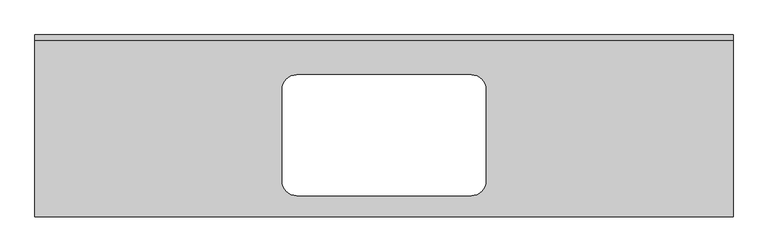
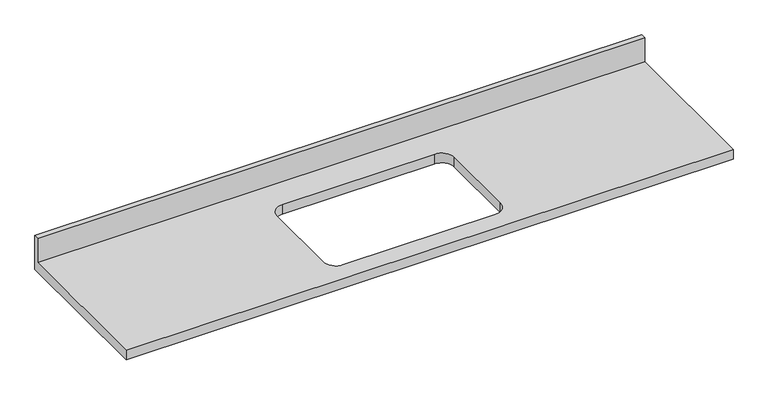
"""IFC4 building model written with IfcOpenShell, lengths in millimetres: furniture geometry, Topo da bancada com pia : Profundidade 600 mm."""

from ifc_helpers import new_model, si_unit, frame, origin, place, context, project, spatial, polyline, circle_curve, source, transform, mapped, element, save
from ifc_brep_helpers import plane_surface, revolved_surface, advanced_brep


def furniture_3e872d23(model_context):
    return source(origin(), model_context, "Body", "AdvancedBrep", [
        advanced_brep(
        [(-1200.4622951, -625.0, 900.0), (1199.5377049, -625.0, 900.0), (1199.5377049, -19.05, 900.0), (-1200.4622951, -19.05, 900.0), (-299.8622951, -137.3, 900.0), (298.9377049, -137.3, 900.0), (349.7377049, -188.1, 900.0), (349.7377049, -501.9, 900.0), (298.9377049, -552.7, 900.0), (-299.8622951, -552.7, 900.0), (-350.6622951, -501.9, 900.0), (-350.6622951, -188.1, 900.0), (1199.5377049, 0.0, 860.0), (1199.5377049, -625.0, 860.0), (-1200.4622951, -625.0, 860.0), (-1200.4622951, 0.0, 860.0), (298.9377049, -137.3, 860.0), (-299.8622951, -137.3, 860.0), (-350.6622951, -188.1, 860.0), (-350.6622951, -501.9, 860.0), (-299.8622951, -552.7, 860.0), (298.9377049, -552.7, 860.0), (349.7377049, -501.9, 860.0), (349.7377049, -188.1, 860.0), (-1200.4622951, 0.0, 1001.6), (1199.5377049, 0.0, 1001.6), (-1200.4622951, -19.05, 1001.6), (1199.5377049, -19.05, 1001.6)],
        [
            (0, 1),
            (1, 2),
            (2, 3),
            (3, 0),
            (4, 5),
            (5, 6, circle_curve(frame((298.9377049, -188.1, 900.0), z_axis=(0.0, 0.0, -1.0), x_axis=(1.0, 0.0, 0.0)), 50.8)),
            (6, 7),
            (7, 8, circle_curve(frame((298.9377049, -501.9, 900.0), z_axis=(0.0, 0.0, -1.0), x_axis=(1.0, 0.0, 0.0)), 50.8)),
            (8, 9),
            (9, 10, circle_curve(frame((-299.8622951, -501.9, 900.0), z_axis=(0.0, 0.0, -1.0), x_axis=(1.0, 0.0, 0.0)), 50.8)),
            (10, 11),
            (11, 4, circle_curve(frame((-299.8622951, -188.1, 900.0), z_axis=(0.0, 0.0, -1.0), x_axis=(1.0, 0.0, 0.0)), 50.8)),
            (12, 13),
            (13, 14),
            (14, 15),
            (15, 12),
            (16, 17),
            (17, 18, circle_curve(frame((-299.8622951, -188.1, 860.0), z_axis=(0.0, 0.0, 1.0), x_axis=(1.0, 0.0, 0.0)), 50.8)),
            (18, 19),
            (19, 20, circle_curve(frame((-299.8622951, -501.9, 860.0), z_axis=(0.0, 0.0, 1.0), x_axis=(1.0, 0.0, 0.0)), 50.8)),
            (20, 21),
            (21, 22, circle_curve(frame((298.9377049, -501.9, 860.0), z_axis=(0.0, 0.0, 1.0), x_axis=(1.0, 0.0, 0.0)), 50.8)),
            (22, 23),
            (23, 16, circle_curve(frame((298.9377049, -188.1, 860.0), z_axis=(0.0, 0.0, 1.0), x_axis=(1.0, 0.0, 0.0)), 50.8)),
            (15, 24),
            (24, 25),
            (25, 12),
            (14, 0),
            (3, 26),
            (26, 24),
            (13, 1),
            (25, 27),
            (27, 2),
            (26, 27),
            (4, 17),
            (16, 5),
            (11, 18),
            (10, 19),
            (9, 20),
            (8, 21),
            (7, 22),
            (6, 23),
        ],
        [
            plane_surface(frame((-1200.4622951, 0.0, 900.0), z_axis=(0.0, 0.0, 1.0), x_axis=(-1.0, 0.0, 0.0))),
            plane_surface(frame((-1200.4622951, 0.0, 860.0), z_axis=(0.0, 0.0, -1.0), x_axis=(1.0, 0.0, 0.0))),
            plane_surface(frame((1199.5377049, 0.0, 900.0), z_axis=(0.0, 1.0, 0.0), x_axis=(0.0, 0.0, -1.0))),
            plane_surface(frame((-1200.4622951, 0.0, 900.0), z_axis=(-1.0, 0.0, 0.0), x_axis=(0.0, 0.0, -1.0))),
            plane_surface(frame((-1200.4622951, -625.0, 900.0), z_axis=(0.0, -1.0, 0.0), x_axis=(0.0, 0.0, -1.0))),
            plane_surface(frame((1199.5377049, -625.0, 900.0), z_axis=(1.0, 0.0, 0.0), x_axis=(0.0, 0.0, -1.0))),
            plane_surface(frame((-1200.4622951, 0.0, 1001.6), z_axis=(0.0, 0.0, 1.0), x_axis=(0.0, -1.0, 0.0))),
            plane_surface(frame((-1200.4622951, -19.05, 1001.6), z_axis=(0.0, -1.0, 0.0), x_axis=(0.0, 0.0, -1.0))),
            plane_surface(frame((298.9377049, -137.3, 900.0), z_axis=(0.0, -1.0, 0.0), x_axis=(0.0, 0.0, -1.0))),
            revolved_surface(polyline([(-249.06229509999997, -188.1, 900.0), (-249.06229509999997, -188.1, 860.0)]), (-299.8622951, -188.1, 860.0), (0.0, 0.0, 1.0)),
            plane_surface(frame((-350.6622951, -188.1, 900.0), z_axis=(1.0, 0.0, 0.0), x_axis=(0.0, 0.0, -1.0))),
            revolved_surface(polyline([(-249.06229509999997, -501.9, 900.0), (-249.06229509999997, -501.9, 860.0)]), (-299.8622951, -501.9, 860.0), (0.0, 0.0, 1.0)),
            plane_surface(frame((-299.8622951, -552.7, 900.0), z_axis=(0.0, 1.0, 0.0), x_axis=(0.0, 0.0, -1.0))),
            revolved_surface(polyline([(349.73770490000004, -501.9, 900.0), (349.73770490000004, -501.9, 860.0)]), (298.9377049, -501.9, 860.0), (0.0, 0.0, 1.0)),
            plane_surface(frame((349.7377049, -501.9, 900.0), z_axis=(-1.0, 0.0, 0.0), x_axis=(0.0, 0.0, -1.0))),
            revolved_surface(polyline([(349.73770490000004, -188.1, 900.0), (349.73770490000004, -188.1, 860.0)]), (298.9377049, -188.1, 860.0), (0.0, 0.0, 1.0)),
        ],
        [
            (0, [[1, 2, 3, 4], [5, 6, 7, 8, 9, 10, 11, 12]]),
            (1, [[13, 14, 15, 16], [17, 18, 19, 20, 21, 22, 23, 24]]),
            (2, [[-16, 25, 26, 27]]),
            (3, [[-15, 28, -4, 29, 30, -25]]),
            (4, [[-1, -28, -14, 31]]),
            (5, [[-13, -27, 32, 33, -2, -31]]),
            (6, [[-30, 34, -32, -26]]),
            (7, [[-34, -29, -3, -33]]),
            (8, [[35, -17, 36, -5]]),
            (9, [[-35, -12, 37, -18]]),
            (10, [[-37, -11, 38, -19]]),
            (11, [[-38, -10, 39, -20]]),
            (12, [[-39, -9, 40, -21]]),
            (13, [[-40, -8, 41, -22]]),
            (14, [[-41, -7, 42, -23]]),
            (15, [[-36, -24, -42, -6]]),
        ],
    ),
    ])


if __name__ == "__main__":
    model = new_model("IFC4")
    model_context = context("Model", 3, world=origin())
    ifc_project = project(units=[si_unit("LENGTHUNIT", "METRE", prefix="MILLI")], contexts=[model_context])
    site = spatial("IfcSite", under=ifc_project)
    building = spatial("IfcBuilding", under=site)
    placement = place(None, origin())
    furniture_shape = furniture_3e872d23(model_context)
    element("IfcFurniture", 1, ObjectType="Topo da bancada com pia : Profundidade 600 mm", at=placement, inside=building, context=model_context, shape_type="MappedRepresentation", body=[
        mapped(furniture_shape, transform((0.0, 0.0, 0.0), x_axis=(1.0, 0.0, 0.0), y_axis=(0.0, 1.0, 0.0), z_axis=(0.0, 0.0, 1.0))),
    ])
    save(model, "model.ifc")

# Revit data of these elements
# Type "Topo da bancada com pia : Profundidade 600 mm"
#   Espessura da bancada = 40 mm
#   Depth = 625 mm
#   Height = 900 mm
#   Comprimento [instance default] = 2500 mm
#   Localização da pia [instance default] = 1200 mm
#   Localização da pia em relação a parede [instance default] = 150 mm
#   Profundidade de abertura da pia [instance default] = 390 mm
#   Largura da abertura da pia [instance default] = 675 mm
#   Material do topo da bancada = none
# Element 1 (IfcFurniture, "Topo da bancada com pia : Profundidade 600 mm")
#   Comprimento = 2400 mm
#   Materials on its faces: "Topo da bancada"
# Materials
#   "Topo da bancada": class "Madeira", colour RGB 226 177 128, transparency 0
